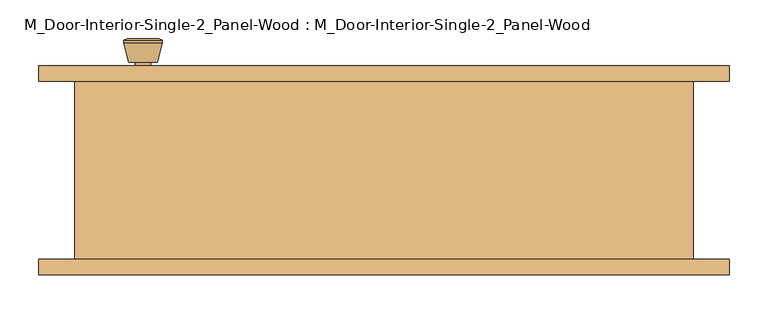
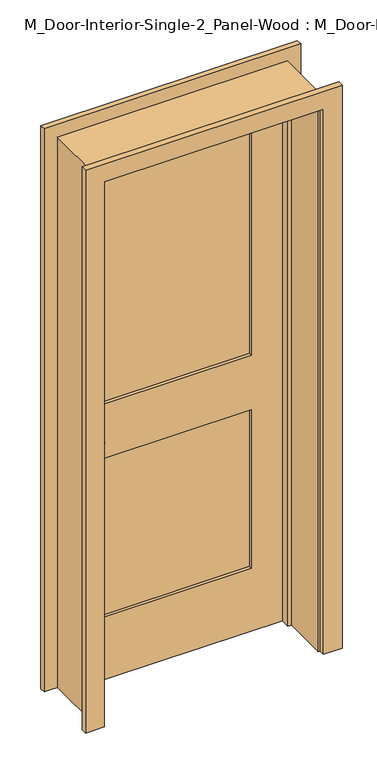
"""IFC4 building model written with IfcOpenShell, lengths in millimetres: door geometry, M_Door-Interior-Single-2_Panel-Wood : M_Door-Interior-Single-2_Panel-Wood."""

from ifc_helpers import new_model, si_unit, point, frame, frame_2d, origin, place, context, project, spatial, polyline, circle_curve, trimmed, segment, composite_curve, outline, extrude, faceted_brep, source, transform, mapped, element, save
from ifc_brep_helpers import plane_surface, cylinder_surface, revolved_surface, advanced_brep


def m_door_interior_single_2_panel_wood_m_door_interior_single_2_fbb4ebeb(model_context):
    return source(origin(), model_context, "Body", "SolidModel", [
        advanced_brep(
        [(-311.5, 70.825, 914.4), (-301.5, 70.825, 914.4), (-321.5, 70.825, 914.4), (-291.0241324, 21.825, 914.4), (-311.5, 21.825, 914.4), (-331.9758676, 21.825, 914.4), (-286.5, 23.6528681, 914.4), (-336.5, 23.6528681, 914.4), (-286.5, 27.1165463, 914.4), (-336.5, 27.1165463, 914.4), (-292.863764, 51.825, 914.4), (-330.136236, 51.825, 914.4), (-301.5, 51.825, 914.4), (-321.5, 51.825, 914.4)],
        [
            (0, 1),
            (1, 2, circle_curve(frame((-311.5, 70.825, 914.4), z_axis=(0.0, 1.0, 0.0), x_axis=(-1.0, 0.0, 0.0)), 10.0)),
            (2, 0),
            (2, 1, circle_curve(frame((-311.5, 70.825, 914.4), z_axis=(0.0, 1.0, 0.0), x_axis=(-1.0, 0.0, 0.0)), 10.0)),
            (3, 4),
            (4, 5),
            (5, 3, circle_curve(frame((-311.5, 21.825, 914.4), z_axis=(0.0, -1.0, 0.0), x_axis=(-1.0, 0.0, 0.0)), 20.4758676)),
            (3, 5, circle_curve(frame((-311.5, 21.825, 914.4), z_axis=(0.0, -1.0, 0.0), x_axis=(-1.0, 0.0, 0.0)), 20.4758676)),
            (6, 3),
            (5, 7),
            (7, 6, circle_curve(frame((-311.5, 23.6528681, 914.4), z_axis=(0.0, -1.0, 0.0), x_axis=(-1.0, 0.0, 0.0)), 25.0)),
            (6, 7, circle_curve(frame((-311.5, 23.6528681, 914.4), z_axis=(0.0, -1.0, 0.0), x_axis=(-1.0, 0.0, 0.0)), 25.0)),
            (8, 6),
            (7, 9),
            (9, 8, circle_curve(frame((-311.5, 27.1165463, 914.4), z_axis=(0.0, -1.0, 0.0), x_axis=(-1.0, 0.0, 0.0)), 25.0)),
            (8, 9, circle_curve(frame((-311.5, 27.1165463, 914.4), z_axis=(0.0, -1.0, 0.0), x_axis=(-1.0, 0.0, 0.0)), 25.0)),
            (10, 8),
            (9, 11),
            (11, 10, circle_curve(frame((-311.5, 51.825, 914.4), z_axis=(0.0, -1.0, 0.0), x_axis=(-1.0, 0.0, 0.0)), 18.636236)),
            (10, 11, circle_curve(frame((-311.5, 51.825, 914.4), z_axis=(0.0, -1.0, 0.0), x_axis=(-1.0, 0.0, 0.0)), 18.636236)),
            (12, 10),
            (11, 13),
            (13, 12, circle_curve(frame((-311.5, 51.825, 914.4), z_axis=(0.0, -1.0, 0.0), x_axis=(-1.0, 0.0, 0.0)), 10.0)),
            (12, 13, circle_curve(frame((-311.5, 51.825, 914.4), z_axis=(0.0, -1.0, 0.0), x_axis=(-1.0, 0.0, 0.0)), 10.0)),
            (1, 12),
            (13, 2),
        ],
        [
            plane_surface(frame((-311.5, 70.825, 914.4), z_axis=(0.0, 1.0, 0.0), x_axis=(-1.0, 0.0, 0.0))),
            plane_surface(frame((-311.5, 21.825, 914.4), z_axis=(0.0, -1.0, 0.0), x_axis=(-1.0, 0.0, 0.0))),
            revolved_surface(polyline([(-331.9758676, 21.825, 914.4), (-336.5, 23.6528681, 914.4)]), (-311.5, 70.825, 914.4), (0.0, 1.0, 0.0)),
            cylinder_surface(frame((-311.5, 70.825, 914.4), z_axis=(0.0, 1.0, 0.0), x_axis=(-1.0, 0.0, 0.0)), 25.0),
            revolved_surface(polyline([(-336.5, 27.1165463, 914.4), (-330.136236, 51.825, 914.4)]), (-311.5, 70.825, 914.4), (0.0, 1.0, 0.0)),
            plane_surface(frame((-311.5, 51.825, 914.4), z_axis=(0.0, 1.0, 0.0), x_axis=(-1.0, 0.0, 0.0))),
            cylinder_surface(frame((-311.5, 70.825, 914.4), z_axis=(0.0, 1.0, 0.0), x_axis=(-1.0, 0.0, 0.0)), 10.0),
        ],
        [
            (0, [[1, 2, 3]]),
            (0, [[-3, 4, -1]]),
            (1, [[5, 6, 7]]),
            (1, [[-6, -5, 8]]),
            (2, [[9, -7, 10, 11]]),
            (2, [[-10, -8, -9, 12]]),
            (3, [[13, -11, 14, 15]]),
            (3, [[-14, -12, -13, 16]]),
            (4, [[17, -15, 18, 19]]),
            (4, [[-18, -16, -17, 20]]),
            (5, [[21, -19, 22, 23]]),
            (5, [[-22, -20, -21, 24]]),
            (6, [[25, -23, 26, -2]]),
            (6, [[-26, -24, -25, -4]]),
        ],
    ),
        extrude(outline(composite_curve([segment(trimmed(circle_curve(frame_2d((914.4, -311.5)), 30.0), [point((914.4, -341.5))], [point((914.4, -281.5))], False, "CARTESIAN"), True, "CONTINUOUS"), segment(trimmed(circle_curve(frame_2d((914.4, -311.5)), 30.0), [point((914.4, -281.5))], [point((914.4, -341.5))], False, "CARTESIAN"), True, "CONTINUOUS")], self_intersect=False)), frame((0.0, 70.825, 0.0), z_axis=(0.0, 1.0, 0.0), x_axis=(0.0, 0.0, 1.0)), (0.0, 0.0, 1.0), 6.0),
        advanced_brep(
        [(-311.5, 117.825, 914.4), (-321.5, 117.825, 914.4), (-301.5, 117.825, 914.4), (-291.0241324, 166.825, 914.4), (-331.9758676, 166.825, 914.4), (-311.5, 166.825, 914.4), (-286.5, 164.9971319, 914.4), (-336.5, 164.9971319, 914.4), (-286.5, 161.5334537, 914.4), (-336.5, 161.5334537, 914.4), (-292.863764, 136.825, 914.4), (-330.136236, 136.825, 914.4), (-301.5, 136.825, 914.4), (-321.5, 136.825, 914.4)],
        [
            (0, 1),
            (1, 2, circle_curve(frame((-311.5, 117.825, 914.4), z_axis=(0.0, -1.0, 0.0), x_axis=(-1.0, 0.0, 0.0)), 10.0)),
            (2, 0),
            (2, 1, circle_curve(frame((-311.5, 117.825, 914.4), z_axis=(0.0, -1.0, 0.0), x_axis=(-1.0, 0.0, 0.0)), 10.0)),
            (3, 4, circle_curve(frame((-311.5, 166.825, 914.4), z_axis=(0.0, 1.0, 0.0), x_axis=(-1.0, 0.0, 0.0)), 20.4758676)),
            (4, 5),
            (5, 3),
            (4, 3, circle_curve(frame((-311.5, 166.825, 914.4), z_axis=(0.0, 1.0, 0.0), x_axis=(-1.0, 0.0, 0.0)), 20.4758676)),
            (6, 7, circle_curve(frame((-311.5, 164.9971319, 914.4), z_axis=(0.0, 1.0, 0.0), x_axis=(-1.0, 0.0, 0.0)), 25.0)),
            (7, 4),
            (3, 6),
            (7, 6, circle_curve(frame((-311.5, 164.9971319, 914.4), z_axis=(0.0, 1.0, 0.0), x_axis=(-1.0, 0.0, 0.0)), 25.0)),
            (8, 9, circle_curve(frame((-311.5, 161.5334537, 914.4), z_axis=(0.0, 1.0, 0.0), x_axis=(-1.0, 0.0, 0.0)), 25.0)),
            (9, 7),
            (6, 8),
            (9, 8, circle_curve(frame((-311.5, 161.5334537, 914.4), z_axis=(0.0, 1.0, 0.0), x_axis=(-1.0, 0.0, 0.0)), 25.0)),
            (10, 11, circle_curve(frame((-311.5, 136.825, 914.4), z_axis=(0.0, 1.0, 0.0), x_axis=(-1.0, 0.0, 0.0)), 18.636236)),
            (11, 9),
            (8, 10),
            (11, 10, circle_curve(frame((-311.5, 136.825, 914.4), z_axis=(0.0, 1.0, 0.0), x_axis=(-1.0, 0.0, 0.0)), 18.636236)),
            (12, 13, circle_curve(frame((-311.5, 136.825, 914.4), z_axis=(0.0, 1.0, 0.0), x_axis=(-1.0, 0.0, 0.0)), 10.0)),
            (13, 11),
            (10, 12),
            (13, 12, circle_curve(frame((-311.5, 136.825, 914.4), z_axis=(0.0, 1.0, 0.0), x_axis=(-1.0, 0.0, 0.0)), 10.0)),
            (1, 13),
            (12, 2),
        ],
        [
            plane_surface(frame((-311.5, 117.825, 914.4), z_axis=(0.0, -1.0, 0.0), x_axis=(-1.0, 0.0, 0.0))),
            plane_surface(frame((-311.5, 166.825, 914.4), z_axis=(0.0, 1.0, 0.0), x_axis=(-1.0, 0.0, 0.0))),
            revolved_surface(polyline([(-331.9758676, 166.825, 914.4), (-336.5, 164.9971319, 914.4)]), (-311.5, 117.825, 914.4), (0.0, -1.0, 0.0)),
            cylinder_surface(frame((-311.5, 117.825, 914.4), z_axis=(0.0, -1.0, 0.0), x_axis=(-1.0, 0.0, 0.0)), 25.0),
            revolved_surface(polyline([(-336.5, 161.5334537, 914.4), (-330.136236, 136.825, 914.4)]), (-311.5, 117.825, 914.4), (0.0, -1.0, 0.0)),
            plane_surface(frame((-311.5, 136.825, 914.4), z_axis=(0.0, -1.0, 0.0), x_axis=(-1.0, 0.0, 0.0))),
            cylinder_surface(frame((-311.5, 117.825, 914.4), z_axis=(0.0, -1.0, 0.0), x_axis=(-1.0, 0.0, 0.0)), 10.0),
        ],
        [
            (0, [[1, 2, 3]]),
            (0, [[-3, 4, -1]]),
            (1, [[5, 6, 7]]),
            (1, [[8, -7, -6]]),
            (2, [[9, 10, -5, 11]]),
            (2, [[12, -11, -8, -10]]),
            (3, [[13, 14, -9, 15]]),
            (3, [[16, -15, -12, -14]]),
            (4, [[17, 18, -13, 19]]),
            (4, [[20, -19, -16, -18]]),
            (5, [[21, 22, -17, 23]]),
            (5, [[24, -23, -20, -22]]),
            (6, [[-2, 25, -21, 26]]),
            (6, [[-4, -26, -24, -25]]),
        ],
    ),
        extrude(outline(composite_curve([segment(trimmed(circle_curve(frame_2d((914.4, -311.5)), 30.0), [point((914.4, -341.5))], [point((914.4, -281.5))], False, "CARTESIAN"), True, "CONTINUOUS"), segment(trimmed(circle_curve(frame_2d((914.4, -311.5)), 30.0), [point((914.4, -281.5))], [point((914.4, -341.5))], False, "CARTESIAN"), True, "CONTINUOUS")], self_intersect=False)), frame((0.0, 111.825, 0.0), z_axis=(0.0, 1.0, 0.0), x_axis=(0.0, 0.0, 1.0)), (0.0, 0.0, 1.0), 6.0),
        extrude(outline(polyline([(255.0, 88.4916667), (-255.0, 88.4916667), (-255.0, 100.1583333), (255.0, 100.1583333), (255.0, 88.4916667)])), frame((0.0, 0.0, 1014.4), z_axis=(0.0, 0.0, 1.0), x_axis=(1.0, 0.0, 0.0)), (0.0, 0.0, 1.0), 865.6),
        extrude(outline(polyline([(255.0, 88.4916667), (-255.0, 88.4916667), (-255.0, 100.1583333), (255.0, 100.1583333), (255.0, 88.4916667)])), frame((0.0, 0.0, 230.0), z_axis=(0.0, 0.0, 1.0), x_axis=(1.0, 0.0, 0.0)), (0.0, 0.0, 1.0), 584.4),
        extrude(outline(polyline([(2000.0, -375.0), (0.0, -375.0), (0.0, 375.0), (2000.0, 375.0), (2000.0, -375.0)]), holes=[polyline([(1880.0, -255.0), (1880.0, 255.0), (1014.4, 255.0), (1014.4, -255.0), (1880.0, -255.0)]), polyline([(814.4, -255.0), (814.4, 255.0), (230.0, 255.0), (230.0, -255.0), (814.4, -255.0)])]), frame((0.0, 76.825, 0.0), z_axis=(0.0, 1.0, 0.0), x_axis=(0.0, 0.0, 1.0)), (0.0, 0.0, 1.0), 35.0),
        faceted_brep([(400.0, 111.825, 0.0), (400.0, -118.175, 0.0), (375.0, -118.175, 0.0), (375.0, 41.9, 0.0), (362.3, 41.9, 0.0), (362.3, 76.825, 0.0), (375.0, 76.825, 0.0), (375.0, 111.825, 0.0), (400.0, 111.825, 2025.0), (400.0, -118.175, 2025.0), (-400.0, -118.175, 2025.0), (-400.0, -118.175, 0.0), (-375.0, -118.175, 0.0), (-375.0, -118.175, 2000.0), (375.0, -118.175, 2000.0), (375.0, 41.9, 2000.0), (-375.0, 41.9, 2000.0), (-375.0, 41.9, 0.0), (-362.3, 41.9, 0.0), (-362.3, 41.9, 1987.3), (362.3, 41.9, 1987.3), (362.3, 76.825, 1987.3), (-362.3, 76.825, 1987.3), (-362.3, 76.825, 0.0), (-375.0, 76.825, 0.0), (-375.0, 76.825, 2000.0), (375.0, 76.825, 2000.0), (375.0, 111.825, 2000.0), (-375.0, 111.825, 2000.0), (-375.0, 111.825, 0.0), (-400.0, 111.825, 0.0), (-400.0, 111.825, 2025.0)], [[[0, 1, 2, 3, 4, 5, 6, 7]], [[1, 0, 8, 9]], [[2, 1, 9, 10, 11, 12, 13, 14]], [[3, 2, 14, 15]], [[4, 3, 15, 16, 17, 18, 19, 20]], [[5, 4, 20, 21]], [[6, 5, 21, 22, 23, 24, 25, 26]], [[7, 6, 26, 27]], [[0, 7, 27, 28, 29, 30, 31, 8]], [[9, 8, 31, 10]], [[15, 14, 13, 16]], [[21, 20, 19, 22]], [[27, 26, 25, 28]], [[30, 29, 24, 23, 18, 17, 12, 11]], [[10, 31, 30, 11]], [[16, 13, 12, 17]], [[22, 19, 18, 23]], [[28, 25, 24, 29]]]),
        extrude(outline(polyline([(0.0, 381.35), (0.0, 446.35), (2071.35, 446.35), (2071.35, -446.35), (0.0, -446.35), (0.0, -381.35), (2006.35, -381.35), (2006.35, 381.35), (0.0, 381.35)])), frame((0.0, -138.175, 0.0), z_axis=(0.0, 1.0, 0.0), x_axis=(0.0, 0.0, 1.0)), (0.0, 0.0, 1.0), 20.0),
        extrude(outline(polyline([(0.0, 381.35), (0.0, 446.35), (2071.35, 446.35), (2071.35, -446.35), (0.0, -446.35), (0.0, -381.35), (2006.35, -381.35), (2006.35, 381.35), (0.0, 381.35)])), frame((0.0, 111.825, 0.0), z_axis=(0.0, 1.0, 0.0), x_axis=(0.0, 0.0, 1.0)), (0.0, 0.0, 1.0), 20.0),
    ])


if __name__ == "__main__":
    model = new_model("IFC4")
    model_context = context("Model", 3, world=origin())
    ifc_project = project(units=[si_unit("LENGTHUNIT", "METRE", prefix="MILLI")], contexts=[model_context])
    site = spatial("IfcSite", under=ifc_project)
    building = spatial("IfcBuilding", under=site)
    placement = place(None, origin())
    m_door_interior_single_2_panel_wood_m_door_interior_single_2_shape = m_door_interior_single_2_panel_wood_m_door_interior_single_2_fbb4ebeb(model_context)
    element("IfcDoor", 1, ObjectType="M_Door-Interior-Single-2_Panel-Wood : M_Door-Interior-Single-2_Panel-Wood", at=placement, inside=building, context=model_context, shape_type="MappedRepresentation", body=[
        mapped(m_door_interior_single_2_panel_wood_m_door_interior_single_2_shape, transform((0.0, 0.0, 0.0), x_axis=(1.0, 0.0, 0.0), y_axis=(0.0, 1.0, 0.0), z_axis=(0.0, 0.0, 1.0))),
    ])
    save(model, "model.ifc")

# Revit data of these elements
# Type "M_Door-Interior-Single-2_Panel-Wood : M_Door-Interior-Single-2_Panel-Wood"
#   Type Mark = "52"
#   Assembly Code = "C1020300"
#   Analytic Construction = "Wooden"
#   Top Rail = 0.12 m
#   Thickness = 0.035 m
#   Thermal Resistance (R) = 0.455703 (m²·K)/W
#   Swing Angle [instance default] = 90.00°
#   Stiles = 0.12 m
#   Rough Width = 0.8 m
#   Rough Height = 2.025 m
#   Lock Rail = 0.2 m
#   Height = 2 m
#   Width = 0.75 m
#   Heat Transfer Coefficient (U) = 2.19465 W/(m²·K)
#   Bottom Rail = 0.23 m
#   Trim Material = Cherry
#   Panel Material = Cherry
#   Frame Material = Cherry
#   Door Handle Material = Aluminum
#   Visual Light Transmittance = 0
#   Solar Heat Gain Coefficient = 0
#   Wall Closure = (empty or 0)
#   Function = (empty or 0)
# Element 1 (IfcDoor, "M_Door-Interior-Single-2_Panel-Wood : M_Door-Interior-Single-2_Panel-Wood")
#   Materials on its faces: "Cherry", "Aluminum"
# Materials
#   "Cherry": class "Wood", colour RGB 226 177 128, transparency 0, Description = "Prunus Serotina", Cost = 0
#   "Aluminum": class "Metal", colour RGB 247 247 247, transparency 0, Description = "Aluminum 6061", Cost = 0
